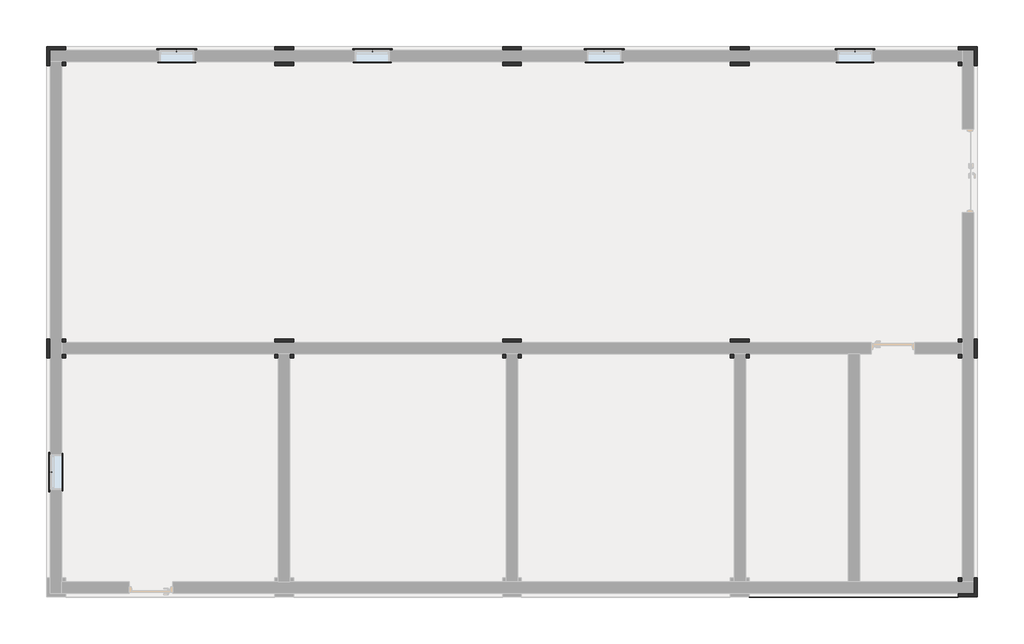
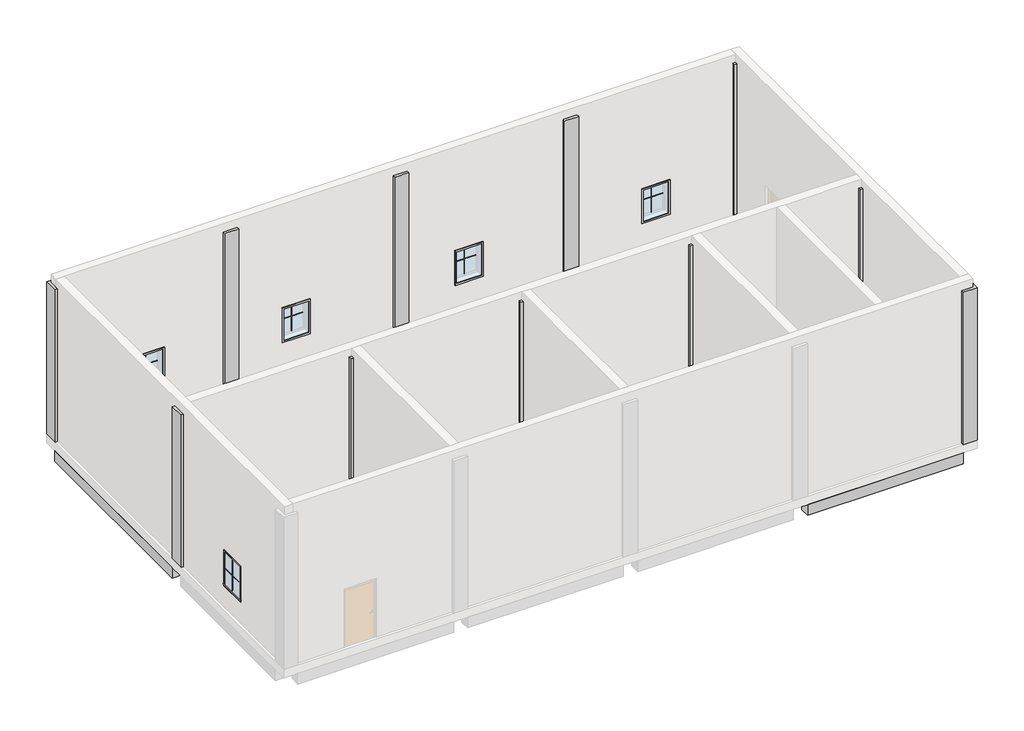
# One storey, part 2 of 2: 15 proxies, 11 columns, 8 beams.
"""IFC4 building model written with IfcOpenShell, lengths in millimetres."""

import ifcopenshell
import ifcopenshell.guid

model = None  # the IFC model being written
_history = None  # IfcOwnerHistory: only IFC2X3 demands one
_inside = {}  # id of a spatial element -> (the spatial element, [elements in it])
_under = {}  # id of a project, library or spatial element -> (it, [spatial elements below it])
_declared = {}  # id of a project -> (the project, [libraries it declares])
_typed = {}  # id of a type object -> (the type object, [elements of that type])
_made_of = {}  # id of a material, layer set ... -> (it, [elements and type objects made of it])


def new_model(schema):
    """Start an empty IFC model of exactly this schema.

    Asked for "IFC4X3", IfcOpenShell would pick the latest addendum, in which some entities
    have other attributes; the version numbers below select the first issue.
    IFC2X3 requires an IfcOwnerHistory on every rooted entity: one is made here for all.
    """
    global model, _history
    if schema == "IFC4X3":
        model = ifcopenshell.file(schema_version=(4, 3, 0, 0))
    else:
        model = ifcopenshell.file(schema=schema)
    _inside.clear()
    _under.clear()
    _declared.clear()
    _typed.clear()
    _made_of.clear()
    _history = None
    if model.schema == "IFC2X3":
        org = make("IfcOrganization", Name="unknown")
        user = make(
            "IfcPersonAndOrganization",
            ThePerson=make("IfcPerson", FamilyName="unknown"),
            TheOrganization=org,
        )
        app = make(
            "IfcApplication",
            ApplicationDeveloper=org,
            Version="unknown",
            ApplicationFullName="unknown",
            ApplicationIdentifier="unknown",
        )
        _history = make(
            "IfcOwnerHistory",
            OwningUser=user,
            OwningApplication=app,
            ChangeAction="ADDED",
            CreationDate=0,
        )
    return model


def make(cls, **values):
    """One entity of the class cls with the attributes given. An attribute that is None is left unset."""
    return model.create_entity(
        cls, **{name: value for name, value in values.items() if value is not None}
    )


def rooted(cls, **values):
    """An entity with a GlobalId (a new one), such as an element, a storey or a relation."""
    return make(cls, GlobalId=ifcopenshell.guid.new(), OwnerHistory=_history, **values)


def si_unit(unit_type, name, prefix=None):
    """IfcSIUnit, for example si_unit("LENGTHUNIT", "METRE", prefix="MILLI")."""
    return make("IfcSIUnit", UnitType=unit_type, Prefix=prefix, Name=name)


def assignment(units):
    """IfcUnitAssignment: the units of a project."""
    return None if units is None else make("IfcUnitAssignment", Units=units)


def point(xyz):
    """IfcCartesianPoint."""
    return None if xyz is None else make("IfcCartesianPoint", Coordinates=xyz)


def direction(xyz):
    """IfcDirection."""
    return None if xyz is None else make("IfcDirection", DirectionRatios=xyz)


def frame(location, z_axis=None, x_axis=None):
    """IfcAxis2Placement3D, a coordinate frame: its origin and axes. An axis left out is left unset."""
    return make(
        "IfcAxis2Placement3D",
        Location=point(location),
        Axis=direction(z_axis),
        RefDirection=direction(x_axis),
    )


def origin():
    """The frame at (0, 0, 0) with its axes left unset."""
    return frame((0.0, 0.0, 0.0))


def origin_with_axes():
    """The frame at (0, 0, 0) with the z axis (0, 0, 1) and the x axis (1, 0, 0) written out."""
    return frame((0.0, 0.0, 0.0), z_axis=(0.0, 0.0, 1.0), x_axis=(1.0, 0.0, 0.0))


def place(relative_to, where):
    """IfcLocalPlacement: puts the frame where relative to a parent placement (None: the world)."""
    return make(
        "IfcLocalPlacement", PlacementRelTo=relative_to, RelativePlacement=where
    )


def context(
    kind, dimensions, precision=None, world=None, true_north=None, identifier=None
):
    """IfcGeometricRepresentationContext, for example the 3D "Model" context."""
    return make(
        "IfcGeometricRepresentationContext",
        ContextIdentifier=identifier,
        ContextType=kind,
        CoordinateSpaceDimension=dimensions,
        Precision=precision,
        WorldCoordinateSystem=world,
        TrueNorth=true_north,
    )


def project(units=None, contexts=None):
    """IfcProject with its units and contexts."""
    return rooted(
        "IfcProject",
        Name="project",
        RepresentationContexts=contexts,
        UnitsInContext=assignment(units),
    )


def spatial(cls, under=None, at=None, **own):
    """A site, building, storey or space (cls), placed at a placement, below another one or the project."""
    s = rooted(cls, ObjectPlacement=at, **own)
    if under is not None:
        _under.setdefault(under.id(), (under, []))[1].append(s)
    return s


def polyline(points):
    """IfcPolyline through the points."""
    return make("IfcPolyline", Points=[point(p) for p in points])


def outline(outer, holes=None, kind="AREA"):
    """IfcArbitraryClosedProfileDef: a profile drawn as a closed curve; with holes, ...WithVoids."""
    if holes is None:
        return make("IfcArbitraryClosedProfileDef", ProfileType=kind, OuterCurve=outer)
    return make(
        "IfcArbitraryProfileDefWithVoids",
        ProfileType=kind,
        OuterCurve=outer,
        InnerCurves=holes,
    )


def extrude(swept, where, along, depth):
    """IfcExtrudedAreaSolid: the profile swept, set in the frame where, extruded along a direction by depth."""
    return make(
        "IfcExtrudedAreaSolid",
        SweptArea=swept,
        Position=where,
        ExtrudedDirection=direction(along),
        Depth=depth,
    )


def faces_of(points, faces, orient=None, outer=None):
    """IfcFace entities. A face is a list of loops; a loop is a list of indices into points, from 0.

    orient and outer hold one flag for each loop. By default every Orientation is true, the
    first loop of a face is its IfcFaceOuterBound and the others are IfcFaceBound.
    """
    made = []
    for i, loops in enumerate(faces):
        bounds = []
        for j, loop in enumerate(loops):
            is_outer = j == 0 if outer is None else outer[i][j]
            bounds.append(
                make(
                    "IfcFaceOuterBound" if is_outer else "IfcFaceBound",
                    Bound=make("IfcPolyLoop", Polygon=[points[k] for k in loop]),
                    Orientation=True if orient is None else orient[i][j],
                )
            )
        made.append(make("IfcFace", Bounds=bounds))
    return made


def faceted_brep(points, faces, orient=None, outer=None, voids=None):
    """IfcFacetedBrep: a solid bounded by flat faces; with voids (closed shells), ...WithVoids."""
    shared = [point(p) for p in points]
    hull = make("IfcClosedShell", CfsFaces=faces_of(shared, faces, orient, outer))
    if voids is None:
        return make("IfcFacetedBrep", Outer=hull)
    return make(
        "IfcFacetedBrepWithVoids",
        Outer=hull,
        Voids=[
            make(cls, CfsFaces=faces_of(shared, fs, o, b)) for cls, fs, o, b in voids
        ],
    )


def shape(context_of_items, identifier, shape_type, items):
    """IfcShapeRepresentation: the items that make up one representation, for example the "Body"."""
    return make(
        "IfcShapeRepresentation",
        ContextOfItems=context_of_items,
        RepresentationIdentifier=identifier,
        RepresentationType=shape_type,
        Items=items,
    )


def source(mapping_origin, context_of_items, identifier, shape_type, items):
    """IfcRepresentationMap: a shape defined once, which mapped items show again and again."""
    return make(
        "IfcRepresentationMap",
        MappingOrigin=mapping_origin,
        MappedRepresentation=shape(context_of_items, identifier, shape_type, items),
    )


def transform(
    local_origin,
    x_axis=None,
    y_axis=None,
    z_axis=None,
    scale=None,
    scale2=None,
    scale3=None,
    uniform=True,
):
    """IfcCartesianTransformationOperator3D, or its non-uniform kind. x_axis, y_axis, z_axis: its Axis1, 2, 3."""
    if uniform:
        return make(
            "IfcCartesianTransformationOperator3D",
            Axis1=direction(x_axis),
            Axis2=direction(y_axis),
            LocalOrigin=point(local_origin),
            Scale=scale,
            Axis3=direction(z_axis),
        )
    return make(
        "IfcCartesianTransformationOperator3DnonUniform",
        Axis1=direction(x_axis),
        Axis2=direction(y_axis),
        LocalOrigin=point(local_origin),
        Scale=scale,
        Axis3=direction(z_axis),
        Scale2=scale2,
        Scale3=scale3,
    )


def mapped(mapping_source, mapping_target):
    """IfcMappedItem: shows the shape of a source again, moved by a transform."""
    return make(
        "IfcMappedItem", MappingSource=mapping_source, MappingTarget=mapping_target
    )


def made_of(thing, what):
    """Note that an element or type object is made of a material, layer set ...; save() writes the relation."""
    if what is not None:
        _made_of.setdefault(what.id(), (what, []))[1].append(thing)
    return thing


def element(
    cls,
    number,
    at=None,
    inside=None,
    cuts=None,
    type_object=None,
    material=None,
    context=None,
    identifier="Body",
    shape_type=None,
    held_by="IfcProductDefinitionShape",
    body=None,
    shapes=None,
    **own,
):
    """One element of the class cls, such as IfcWall. Its Tag is "e" and its number.

    at: its placement. inside: the storey or other place that contains it. cuts: it is an
    opening in that element (IfcRelVoidsElement). A single representation is given by context,
    identifier, shape_type and body (its items); several are given by shapes. held_by: the class
    of the entity that holds the representations. save() writes the other relations.
    """
    e = rooted(cls, Tag="e%d" % number, ObjectPlacement=at, **own)
    if body is not None:
        shapes = [shape(context, identifier, shape_type, body)]
    if shapes is not None:
        e.Representation = make(held_by, Representations=shapes)
    if inside is not None:
        _inside.setdefault(inside.id(), (inside, []))[1].append(e)
    if cuts is not None:
        rooted(
            "IfcRelVoidsElement", RelatingBuildingElement=cuts, RelatedOpeningElement=e
        )
    if type_object is not None:
        _typed.setdefault(type_object.id(), (type_object, []))[1].append(e)
    return made_of(e, material)


def aggregate(whole, parts):
    """IfcRelAggregates: a whole, such as a stair, and the parts it consists of."""
    return rooted("IfcRelAggregates", RelatingObject=whole, RelatedObjects=parts)


def save(model, path):
    """Write the relations noted so far, then the file.

    IfcRelAggregates (storeys below a building ...), IfcRelContainedInSpatialStructure (elements
    in a storey), IfcRelDefinesByType, IfcRelAssociatesMaterial and IfcRelDeclares: one each for
    every whole, place, type object, material and project.
    """
    for whole, parts in _under.values():
        aggregate(whole, parts)
    for where, things in _inside.values():
        rooted(
            "IfcRelContainedInSpatialStructure",
            RelatedElements=things,
            RelatingStructure=where,
        )
    for kind, things in _typed.values():
        rooted("IfcRelDefinesByType", RelatedObjects=things, RelatingType=kind)
    for what, things in _made_of.values():
        rooted("IfcRelAssociatesMaterial", RelatedObjects=things, RelatingMaterial=what)
    for by, libraries in _declared.values():
        rooted("IfcRelDeclares", RelatingContext=by, RelatedDefinitions=libraries)
    model.write(path)


def m_muntin_pattern_2x2_m_muntin_pattern_2x2_ad852c99(model_context):
    return source(origin(), model_context, "Body", "SweptSolid", [
        extrude(outline(polyline([(568.25, -6.35), (568.25, -411.9), (555.55, -411.9), (555.55, -6.35), (0.0, -6.35), (0.0, 6.35), (555.55, 6.35), (555.55, 411.9), (568.25, 411.9), (568.25, 6.35), (1123.8, 6.35), (1123.8, -6.35), (568.25, -6.35)])), frame((0.0, -22.225, 0.0), z_axis=(0.0, 1.0, 0.0), x_axis=(0.0, 0.0, 1.0)), (0.0, 0.0, 1.0), 12.7),
        extrude(outline(polyline([(568.25, -6.35), (568.25, -411.9), (555.55, -411.9), (555.55, -6.35), (0.0, -6.35), (0.0, 6.35), (555.55, 6.35), (555.55, 411.9), (568.25, 411.9), (568.25, 6.35), (1123.8, 6.35), (1123.8, -6.35), (568.25, -6.35)])), frame((0.0, 9.525, 0.0), z_axis=(0.0, 1.0, 0.0), x_axis=(0.0, 0.0, 1.0)), (0.0, 0.0, 1.0), 12.7),
    ])


def m_trim_window_exterior_flat_with_sill_71544b40(model_context):
    return source(origin(), model_context, "Body", "SweptSolid", [
        extrude(outline(polyline([(510.0, -1220.4323709), (510.0, -1280.4323709), (-510.0, -1280.4323709), (-510.0, -1220.4323709), (510.0, -1220.4323709)])), origin_with_axes(), (0.0, 0.0, 1.0), 19.05),
        extrude(outline(polyline([(-1230.0, 38.1), (-1202.4580645, 38.1), (-1200.0, 19.05), (-1200.0, 0.0), (-1220.4323709, 0.0), (-1220.4323709, 19.05), (-1230.0, 19.05), (-1230.0, 38.1)])), frame((-522.7, 0.0, 0.0), z_axis=(1.0, 0.0, 0.0), x_axis=(0.0, 1.0, 0.0)), (0.0, 0.0, 1.0), 1045.4),
        extrude(outline(polyline([(-510.0, 60.0), (510.0, 60.0), (510.0, -1200.0), (450.0, -1200.0), (450.0, 0.0), (-450.0, 0.0), (-450.0, -1200.0), (-510.0, -1200.0), (-510.0, 60.0)])), origin_with_axes(), (0.0, 0.0, 1.0), 19.05),
    ])


def m_trim_window_interior_flat_picture_frame_24fe8ef8(model_context):
    return source(origin(), model_context, "Body", "SweptSolid", [
        extrude(outline(polyline([(497.3, 47.3), (497.3, -1247.3), (-497.3, -1247.3), (-497.3, 47.3), (497.3, 47.3)]), holes=[polyline([(437.3, -12.7), (-437.3, -12.7), (-437.3, -1187.3), (437.3, -1187.3), (437.3, -12.7)])]), origin_with_axes(), (0.0, 0.0, 1.0), 30.0),
    ])


model = new_model("IFC4")

# Units and contexts
model_context = context("Model", 3, world=origin())
ifc_project = project(units=[si_unit("LENGTHUNIT", "METRE", prefix="MILLI")], contexts=[model_context])

# Site, building, storey
site = spatial("IfcSite", under=ifc_project)
building = spatial("IfcBuilding", under=site)
storey = spatial("IfcBuildingStorey", under=building, Name="1st FL GL+200", Elevation=0.0)

# Beams
placement = place(None, origin())
element("IfcBeam", 1, ObjectType="RC Beam_Rectangular : 350 x 700mm", at=placement, inside=storey, context=model_context, shape_type="SweptSolid", body=[
    extrude(outline(polyline([(5204.2726763, 1485.9763125), (5554.2726763, 1485.9763125), (5554.2726763, -4314.0236875), (5204.2726763, -4314.0236875), (5204.2726763, 1485.9763125)])), frame((0.0, 0.0, -700.0), z_axis=(0.0, 0.0, 1.0), x_axis=(1.0, 0.0, 0.0)), (0.0, 0.0, 1.0), 400.0),
])
element("IfcBeam", 2, ObjectType="RC Beam_Rectangular : 350 x 700mm", at=placement, inside=storey, context=model_context, shape_type="SweptSolid", body=[
    extrude(outline(polyline([(5554.2726763, 1998.6763125), (5204.2726763, 1998.6763125), (5204.2726763, 9185.9763125), (5554.2726763, 9185.9763125), (5554.2726763, 1998.6763125)])), frame((0.0, 0.0, -700.0), z_axis=(0.0, 0.0, 1.0), x_axis=(1.0, 0.0, 0.0)), (0.0, 0.0, 1.0), 400.0),
])
element("IfcBeam", 3, ObjectType="RC Beam_Rectangular : 350 x 700mm", at=placement, inside=storey, context=model_context, shape_type="SweptSolid", body=[
    extrude(outline(polyline([(-18595.7273237, 1998.6763125), (-18945.7273237, 1998.6763125), (-18945.7273237, 9185.9763125), (-18595.7273237, 9185.9763125), (-18595.7273237, 1998.6763125)])), frame((0.0, 0.0, -700.0), z_axis=(0.0, 0.0, 1.0), x_axis=(1.0, 0.0, 0.0)), (0.0, 0.0, 1.0), 400.0),
])
element("IfcBeam", 4, ObjectType="RC Beam_Rectangular : 350 x 700mm", at=placement, inside=storey, context=model_context, shape_type="SweptSolid", body=[
    extrude(outline(polyline([(-12945.7273237, 9685.9763125), (-12945.7273237, 9335.9763125), (-18445.7273237, 9335.9763125), (-18445.7273237, 9685.9763125), (-12945.7273237, 9685.9763125)])), frame((0.0, 0.0, -700.0), z_axis=(0.0, 0.0, 1.0), x_axis=(1.0, 0.0, 0.0)), (0.0, 0.0, 1.0), 400.0),
])
element("IfcBeam", 5, ObjectType="RC Beam_Rectangular : 350 x 700mm", at=placement, inside=storey, context=model_context, shape_type="SweptSolid", body=[
    extrude(outline(polyline([(-12433.0273237, 9335.9763125), (-12433.0273237, 9685.9763125), (-6945.7273237, 9685.9763125), (-6945.7273237, 9335.9763125), (-12433.0273237, 9335.9763125)])), frame((0.0, 0.0, -700.0), z_axis=(0.0, 0.0, 1.0), x_axis=(1.0, 0.0, 0.0)), (0.0, 0.0, 1.0), 400.0),
])
element("IfcBeam", 6, ObjectType="RC Beam_Rectangular : 350 x 700mm", at=placement, inside=storey, context=model_context, shape_type="SweptSolid", body=[
    extrude(outline(polyline([(-6433.0273237, 9335.9763125), (-6433.0273237, 9685.9763125), (-945.7273237, 9685.9763125), (-945.7273237, 9335.9763125), (-6433.0273237, 9335.9763125)])), frame((0.0, 0.0, -700.0), z_axis=(0.0, 0.0, 1.0), x_axis=(1.0, 0.0, 0.0)), (0.0, 0.0, 1.0), 400.0),
])
element("IfcBeam", 7, ObjectType="RC Beam_Rectangular : 350 x 700mm", at=placement, inside=storey, context=model_context, shape_type="SweptSolid", body=[
    extrude(outline(polyline([(-433.0273237, 9335.9763125), (-433.0273237, 9685.9763125), (5054.2726763, 9685.9763125), (5054.2726763, 9335.9763125), (-433.0273237, 9335.9763125)])), frame((0.0, 0.0, -700.0), z_axis=(0.0, 0.0, 1.0), x_axis=(1.0, 0.0, 0.0)), (0.0, 0.0, 1.0), 400.0),
])
element("IfcBeam", 8, ObjectType="RC Beam_Rectangular : 350 x 700mm", at=placement, inside=storey, context=model_context, shape_type="SweptSolid", body=[
    extrude(outline(polyline([(5054.2726763, -4464.0236875), (5054.2726763, -4814.0236875), (-445.7273237, -4814.0236875), (-445.7273237, -4464.0236875), (5054.2726763, -4464.0236875)])), frame((0.0, 0.0, -700.0), z_axis=(0.0, 0.0, 1.0), x_axis=(1.0, 0.0, 0.0)), (0.0, 0.0, 1.0), 400.0),
])

# Proxies
m_muntin_pattern_2x2_m_muntin_pattern_2x2_shape = m_muntin_pattern_2x2_m_muntin_pattern_2x2_ad852c99(model_context)
element("IfcBuildingElementProxy", 9, Name="M_Muntin Pattern_2x2 : M_Muntin Pattern_2x2", ObjectType="M_Muntin Pattern_2x2 : M_Muntin Pattern_2x2", at=placement, inside=storey, context=model_context, shape_type="MappedRepresentation", body=[
    mapped(m_muntin_pattern_2x2_m_muntin_pattern_2x2_shape, transform((2329.2726763, 9576.4513125, 938.1), x_axis=(-1.0, 0.0, 0.0), y_axis=(0.0, -1.0, 0.0), z_axis=(0.0, 0.0, 1.0))),
])
element("IfcBuildingElementProxy", 10, Name="M_Muntin Pattern_2x2 : M_Muntin Pattern_2x2", ObjectType="M_Muntin Pattern_2x2 : M_Muntin Pattern_2x2", at=placement, inside=storey, context=model_context, shape_type="MappedRepresentation", body=[
    mapped(m_muntin_pattern_2x2_m_muntin_pattern_2x2_shape, transform((-4270.7273237, 9576.4513125, 938.1), x_axis=(-1.0, 0.0, 0.0), y_axis=(0.0, -1.0, 0.0), z_axis=(0.0, 0.0, 1.0))),
])
element("IfcBuildingElementProxy", 11, Name="M_Muntin Pattern_2x2 : M_Muntin Pattern_2x2", ObjectType="M_Muntin Pattern_2x2 : M_Muntin Pattern_2x2", at=placement, inside=storey, context=model_context, shape_type="MappedRepresentation", body=[
    mapped(m_muntin_pattern_2x2_m_muntin_pattern_2x2_shape, transform((-10370.7273237, 9576.4513125, 938.1), x_axis=(-1.0, 0.0, 0.0), y_axis=(0.0, -1.0, 0.0), z_axis=(0.0, 0.0, 1.0))),
])
element("IfcBuildingElementProxy", 12, Name="M_Muntin Pattern_2x2 : M_Muntin Pattern_2x2", ObjectType="M_Muntin Pattern_2x2 : M_Muntin Pattern_2x2", at=placement, inside=storey, context=model_context, shape_type="MappedRepresentation", body=[
    mapped(m_muntin_pattern_2x2_m_muntin_pattern_2x2_shape, transform((-15520.7273237, 9576.4513125, 938.1), x_axis=(-1.0, 0.0, 0.0), y_axis=(0.0, -1.0, 0.0), z_axis=(0.0, 0.0, 1.0))),
])
element("IfcBuildingElementProxy", 13, Name="M_Muntin Pattern_2x2 : M_Muntin Pattern_2x2", ObjectType="M_Muntin Pattern_2x2 : M_Muntin Pattern_2x2", at=placement, inside=storey, context=model_context, shape_type="MappedRepresentation", body=[
    mapped(m_muntin_pattern_2x2_m_muntin_pattern_2x2_shape, transform((-18836.2023237, -1526.5236875, 938.1), x_axis=(0.0, -1.0, 0.0), y_axis=(1.0, 0.0, 0.0), z_axis=(0.0, 0.0, 1.0))),
])
m_trim_window_exterior_flat_with_sill_shape = m_trim_window_exterior_flat_with_sill_71544b40(model_context)
element("IfcBuildingElementProxy", 14, Name="M_Trim-Window-Exterior-Flat : with Sill", ObjectType="M_Trim-Window-Exterior-Flat : with Sill", at=placement, inside=storey, context=model_context, shape_type="MappedRepresentation", body=[
    mapped(m_trim_window_exterior_flat_with_sill_shape, transform((2329.2726763, 9585.9763125, 2100.0), x_axis=(-1.0, 0.0, 0.0), y_axis=(0.0, 0.0, 1.0), z_axis=(0.0, 1.0, 0.0))),
])
element("IfcBuildingElementProxy", 15, Name="M_Trim-Window-Exterior-Flat : with Sill", ObjectType="M_Trim-Window-Exterior-Flat : with Sill", at=placement, inside=storey, context=model_context, shape_type="MappedRepresentation", body=[
    mapped(m_trim_window_exterior_flat_with_sill_shape, transform((-4270.7273237, 9585.9763125, 2100.0), x_axis=(-1.0, 0.0, 0.0), y_axis=(0.0, 0.0, 1.0), z_axis=(0.0, 1.0, 0.0))),
])
element("IfcBuildingElementProxy", 16, Name="M_Trim-Window-Exterior-Flat : with Sill", ObjectType="M_Trim-Window-Exterior-Flat : with Sill", at=placement, inside=storey, context=model_context, shape_type="MappedRepresentation", body=[
    mapped(m_trim_window_exterior_flat_with_sill_shape, transform((-10370.7273237, 9585.9763125, 2100.0), x_axis=(-1.0, 0.0, 0.0), y_axis=(0.0, 0.0, 1.0), z_axis=(0.0, 1.0, 0.0))),
])
element("IfcBuildingElementProxy", 17, Name="M_Trim-Window-Exterior-Flat : with Sill", ObjectType="M_Trim-Window-Exterior-Flat : with Sill", at=placement, inside=storey, context=model_context, shape_type="MappedRepresentation", body=[
    mapped(m_trim_window_exterior_flat_with_sill_shape, transform((-15520.7273237, 9585.9763125, 2100.0), x_axis=(-1.0, 0.0, 0.0), y_axis=(0.0, 0.0, 1.0), z_axis=(0.0, 1.0, 0.0))),
])
element("IfcBuildingElementProxy", 18, Name="M_Trim-Window-Exterior-Flat : with Sill", ObjectType="M_Trim-Window-Exterior-Flat : with Sill", at=placement, inside=storey, context=model_context, shape_type="MappedRepresentation", body=[
    mapped(m_trim_window_exterior_flat_with_sill_shape, transform((-18845.7273237, -1526.5236875, 2100.0), x_axis=(0.0, -1.0, 0.0), y_axis=(0.0, 0.0, 1.0), z_axis=(-1.0, 0.0, 0.0))),
])
m_trim_window_interior_flat_picture_frame_shape = m_trim_window_interior_flat_picture_frame_24fe8ef8(model_context)
element("IfcBuildingElementProxy", 19, Name="M_Trim-Window-Interior-Flat : Picture Frame", ObjectType="M_Trim-Window-Interior-Flat : Picture Frame", at=placement, inside=storey, context=model_context, shape_type="MappedRepresentation", body=[
    mapped(m_trim_window_interior_flat_picture_frame_shape, transform((2329.2726763, 9285.9763125, 2100.0), x_axis=(1.0, 0.0, 0.0), y_axis=(0.0, 0.0, 1.0), z_axis=(0.0, -1.0, 0.0))),
])
element("IfcBuildingElementProxy", 20, Name="M_Trim-Window-Interior-Flat : Picture Frame", ObjectType="M_Trim-Window-Interior-Flat : Picture Frame", at=placement, inside=storey, context=model_context, shape_type="MappedRepresentation", body=[
    mapped(m_trim_window_interior_flat_picture_frame_shape, transform((-4270.7273237, 9285.9763125, 2100.0), x_axis=(1.0, 0.0, 0.0), y_axis=(0.0, 0.0, 1.0), z_axis=(0.0, -1.0, 0.0))),
])
element("IfcBuildingElementProxy", 21, Name="M_Trim-Window-Interior-Flat : Picture Frame", ObjectType="M_Trim-Window-Interior-Flat : Picture Frame", at=placement, inside=storey, context=model_context, shape_type="MappedRepresentation", body=[
    mapped(m_trim_window_interior_flat_picture_frame_shape, transform((-10370.7273237, 9285.9763125, 2100.0), x_axis=(1.0, 0.0, 0.0), y_axis=(0.0, 0.0, 1.0), z_axis=(0.0, -1.0, 0.0))),
])
element("IfcBuildingElementProxy", 22, Name="M_Trim-Window-Interior-Flat : Picture Frame", ObjectType="M_Trim-Window-Interior-Flat : Picture Frame", at=placement, inside=storey, context=model_context, shape_type="MappedRepresentation", body=[
    mapped(m_trim_window_interior_flat_picture_frame_shape, transform((-15520.7273237, 9285.9763125, 2100.0), x_axis=(1.0, 0.0, 0.0), y_axis=(0.0, 0.0, 1.0), z_axis=(0.0, -1.0, 0.0))),
])
element("IfcBuildingElementProxy", 23, Name="M_Trim-Window-Interior-Flat : Picture Frame", ObjectType="M_Trim-Window-Interior-Flat : Picture Frame", at=placement, inside=storey, context=model_context, shape_type="MappedRepresentation", body=[
    mapped(m_trim_window_interior_flat_picture_frame_shape, transform((-18545.7273237, -1526.5236875, 2100.0), x_axis=(0.0, 1.0, 0.0), y_axis=(0.0, 0.0, 1.0), z_axis=(1.0, 0.0, 0.0))),
])

# Columns
element("IfcColumn", 24, ObjectType="RC_Column_Rectangular : 500 x 500mm", at=placement, inside=storey, context=model_context, shape_type="Brep", body=[
    faceted_brep([(-18945.7273237, 9185.9763125, 0.0), (-18945.7273237, 9685.9763125, 0.0), (-18445.7273237, 9685.9763125, 0.0), (-18445.7273237, 9585.9763125, 0.0), (-18845.7273237, 9585.9763125, 0.0), (-18845.7273237, 9285.9763125, 0.0), (-18845.7273237, 9185.9763125, 0.0), (-18945.7273237, 9685.9763125, 5700.0), (-18445.7273237, 9685.9763125, 5700.0), (-18445.7273237, 9685.9763125, 5300.0), (-18945.7273237, 9185.9763125, 5300.0), (-18945.7273237, 9185.9763125, 5700.0), (-18845.7273237, 9185.9763125, 5300.0), (-18845.7273237, 9185.9763125, 5700.0), (-18445.7273237, 9585.9763125, 5700.0), (-18445.7273237, 9585.9763125, 5300.0), (-18845.7273237, 9585.9763125, 5700.0)], [[[0, 1, 2, 3, 4, 5, 6]], [[2, 1, 7, 8, 9]], [[1, 0, 10, 11, 7]], [[11, 10, 0, 6, 12, 13]], [[2, 9, 8, 14, 15, 3]], [[16, 4, 3, 15, 14]], [[4, 16, 13, 12, 6, 5]], [[8, 7, 11, 13, 16, 14]]]),
    faceted_brep([(-18445.7273237, 9185.9763125, 5700.0), (-18445.7273237, 9285.9763125, 5700.0), (-18545.7273237, 9285.9763125, 5700.0), (-18545.7273237, 9185.9763125, 5700.0), (-18445.7273237, 9285.9763125, 0.0), (-18545.7273237, 9285.9763125, 0.0), (-18445.7273237, 9185.9763125, 0.0), (-18545.7273237, 9185.9763125, 0.0)], [[[0, 1, 2, 3]], [[1, 4, 5, 2]], [[0, 6, 4, 1]], [[5, 7, 3, 2]], [[4, 6, 7, 5]], [[6, 0, 3, 7]]]),
])
element("IfcColumn", 25, ObjectType="RC_Column_Rectangular : 500 x 500mm", at=placement, inside=storey, context=model_context, shape_type="Brep", body=[
    faceted_brep([(-18945.7273237, 1485.9763125, 0.0), (-18945.7273237, 1985.9763125, 0.0), (-18845.7273237, 1985.9763125, 0.0), (-18845.7273237, 1485.9763125, 0.0), (-18945.7273237, 1485.9763125, 5300.0), (-18945.7273237, 1485.9763125, 5700.0), (-18945.7273237, 1985.9763125, 5700.0), (-18945.7273237, 1985.9763125, 5300.0), (-18845.7273237, 1485.9763125, 5300.0), (-18845.7273237, 1485.9763125, 5700.0), (-18845.7273237, 1985.9763125, 5300.0), (-18845.7273237, 1985.9763125, 5700.0)], [[[0, 1, 2, 3]], [[1, 0, 4, 5, 6, 7]], [[5, 4, 0, 3, 8, 9]], [[3, 2, 10, 11, 9, 8]], [[1, 7, 6, 11, 10, 2]], [[6, 5, 9, 11]]]),
    faceted_brep([(-18445.7273237, 1985.9763125, 5700.0), (-18445.7273237, 1985.9763125, 0.0), (-18545.7273237, 1985.9763125, 0.0), (-18545.7273237, 1985.9763125, 5700.0), (-18445.7273237, 1910.9763125, 5700.0), (-18445.7273237, 1885.9763125, 5700.0), (-18445.7273237, 1885.9763125, 5300.0), (-18445.7273237, 1885.9763125, 0.0), (-18545.7273237, 1885.9763125, 0.0), (-18545.7273237, 1885.9763125, 5700.0)], [[[0, 1, 2, 3]], [[1, 0, 4, 5, 6, 7]], [[2, 1, 7, 8]], [[7, 6, 5, 9, 8]], [[0, 3, 9, 5, 4]], [[3, 2, 8, 9]]]),
    faceted_brep([(-18545.7273237, 1485.9763125, 5700.0), (-18445.7273237, 1485.9763125, 5700.0), (-18445.7273237, 1560.9763125, 5700.0), (-18445.7273237, 1585.9763125, 5700.0), (-18545.7273237, 1585.9763125, 5700.0), (-18545.7273237, 1485.9763125, 0.0), (-18545.7273237, 1585.9763125, 0.0), (-18445.7273237, 1485.9763125, 0.0), (-18445.7273237, 1585.9763125, 5300.0), (-18445.7273237, 1585.9763125, 0.0)], [[[0, 1, 2, 3, 4]], [[5, 0, 4, 6]], [[7, 1, 0, 5]], [[3, 8, 9, 6, 4]], [[1, 7, 9, 8, 3, 2]], [[7, 5, 6, 9]]]),
])
element("IfcColumn", 26, ObjectType="RC_Column_Rectangular : 500 x 500mm", at=placement, inside=storey, context=model_context, shape_type="Brep", body=[
    faceted_brep([(-12945.7273237, 9685.9763125, 0.0), (-12445.7273237, 9685.9763125, 0.0), (-12445.7273237, 9585.9763125, 0.0), (-12945.7273237, 9585.9763125, 0.0), (-12945.7273237, 9685.9763125, 5300.0), (-12945.7273237, 9685.9763125, 5700.0), (-12445.7273237, 9685.9763125, 5700.0), (-12945.7273237, 9585.9763125, 5300.0), (-12945.7273237, 9585.9763125, 5700.0), (-12445.7273237, 9585.9763125, 5700.0)], [[[0, 1, 2, 3]], [[1, 0, 4, 5, 6]], [[5, 4, 0, 3, 7, 8]], [[1, 6, 9, 2]], [[3, 2, 9, 8, 7]], [[6, 5, 8, 9]]]),
    faceted_brep([(-12945.7273237, 9185.9763125, 0.0), (-12445.7273237, 9185.9763125, 0.0), (-12445.7273237, 9185.9763125, 5700.0), (-12520.7273237, 9185.9763125, 5700.0), (-12870.7273237, 9185.9763125, 5700.0), (-12945.7273237, 9185.9763125, 5700.0), (-12445.7273237, 9285.9763125, 5700.0), (-12945.7273237, 9285.9763125, 5700.0), (-12445.7273237, 9285.9763125, 0.0), (-12945.7273237, 9285.9763125, 0.0)], [[[0, 1, 2, 3, 4, 5]], [[5, 4, 3, 2, 6, 7]], [[8, 9, 7, 6]], [[1, 0, 9, 8]], [[0, 5, 7, 9]], [[2, 1, 8, 6]]]),
])
element("IfcColumn", 27, ObjectType="RC_Column_Rectangular : 500 x 500mm", at=placement, inside=storey, context=model_context, shape_type="Brep", body=[
    faceted_brep([(-12945.7273237, 1985.9763125, 0.0), (-12445.7273237, 1985.9763125, 0.0), (-12445.7273237, 1885.9763125, 0.0), (-12945.7273237, 1885.9763125, 0.0), (-12945.7273237, 1985.9763125, 5700.0), (-12870.7273237, 1985.9763125, 5700.0), (-12520.7273237, 1985.9763125, 5700.0), (-12445.7273237, 1985.9763125, 5700.0), (-12945.7273237, 1885.9763125, 5300.0), (-12945.7273237, 1885.9763125, 5700.0), (-12945.7273237, 1910.9763125, 5700.0), (-12445.7273237, 1910.9763125, 5700.0), (-12445.7273237, 1885.9763125, 5700.0), (-12445.7273237, 1885.9763125, 5300.0)], [[[0, 1, 2, 3]], [[1, 0, 4, 5, 6, 7]], [[4, 0, 3, 8, 9, 10]], [[1, 7, 11, 12, 13, 2]], [[3, 2, 13, 12, 9, 8]], [[7, 6, 5, 4, 10, 9, 12, 11]]]),
    faceted_brep([(-12945.7273237, 1485.9763125, 5700.0), (-12945.7273237, 1485.9763125, 0.0), (-12845.7273237, 1485.9763125, 0.0), (-12845.7273237, 1485.9763125, 5300.0), (-12845.7273237, 1485.9763125, 5700.0), (-12870.7273237, 1485.9763125, 5700.0), (-12945.7273237, 1585.9763125, 0.0), (-12945.7273237, 1585.9763125, 5300.0), (-12945.7273237, 1585.9763125, 5700.0), (-12845.7273237, 1585.9763125, 5700.0), (-12845.7273237, 1585.9763125, 0.0), (-12945.7273237, 1560.9763125, 5700.0)], [[[0, 1, 2, 3, 4, 5]], [[6, 7, 8, 9, 10]], [[1, 6, 10, 2]], [[1, 0, 11, 8, 7, 6]], [[4, 3, 2, 10, 9]], [[8, 11, 0, 5, 4, 9]]]),
    faceted_brep([(-12445.7273237, 1485.9763125, 5700.0), (-12445.7273237, 1560.9763125, 5700.0), (-12445.7273237, 1585.9763125, 5700.0), (-12545.7273237, 1585.9763125, 5700.0), (-12545.7273237, 1485.9763125, 5700.0), (-12520.7273237, 1485.9763125, 5700.0), (-12445.7273237, 1485.9763125, 0.0), (-12445.7273237, 1585.9763125, 0.0), (-12445.7273237, 1585.9763125, 5300.0), (-12545.7273237, 1485.9763125, 0.0), (-12545.7273237, 1485.9763125, 5300.0), (-12545.7273237, 1585.9763125, 0.0)], [[[0, 1, 2, 3, 4, 5]], [[0, 6, 7, 8, 2, 1]], [[9, 10, 4, 3, 11]], [[6, 0, 5, 4, 10, 9]], [[2, 8, 7, 11, 3]], [[7, 6, 9, 11]]]),
])
element("IfcColumn", 28, ObjectType="RC_Column_Rectangular : 500 x 500mm", at=placement, inside=storey, context=model_context, shape_type="Brep", body=[
    faceted_brep([(-6945.7273237, 9685.9763125, 0.0), (-6445.7273237, 9685.9763125, 0.0), (-6445.7273237, 9585.9763125, 0.0), (-6945.7273237, 9585.9763125, 0.0), (-6945.7273237, 9685.9763125, 5300.0), (-6945.7273237, 9685.9763125, 5700.0), (-6445.7273237, 9685.9763125, 5700.0), (-6945.7273237, 9585.9763125, 5300.0), (-6945.7273237, 9585.9763125, 5700.0), (-6445.7273237, 9585.9763125, 5700.0)], [[[0, 1, 2, 3]], [[1, 0, 4, 5, 6]], [[5, 4, 0, 3, 7, 8]], [[1, 6, 9, 2]], [[3, 2, 9, 8, 7]], [[6, 5, 8, 9]]]),
    faceted_brep([(-6945.7273237, 9185.9763125, 0.0), (-6445.7273237, 9185.9763125, 0.0), (-6445.7273237, 9185.9763125, 5700.0), (-6520.7273237, 9185.9763125, 5700.0), (-6870.7273237, 9185.9763125, 5700.0), (-6945.7273237, 9185.9763125, 5700.0), (-6445.7273237, 9285.9763125, 5700.0), (-6945.7273237, 9285.9763125, 5700.0), (-6445.7273237, 9285.9763125, 0.0), (-6945.7273237, 9285.9763125, 0.0)], [[[0, 1, 2, 3, 4, 5]], [[5, 4, 3, 2, 6, 7]], [[8, 9, 7, 6]], [[1, 0, 9, 8]], [[0, 5, 7, 9]], [[2, 1, 8, 6]]]),
])
element("IfcColumn", 29, ObjectType="RC_Column_Rectangular : 500 x 500mm", at=placement, inside=storey, context=model_context, shape_type="Brep", body=[
    faceted_brep([(-6945.7273237, 1985.9763125, 0.0), (-6445.7273237, 1985.9763125, 0.0), (-6445.7273237, 1885.9763125, 0.0), (-6945.7273237, 1885.9763125, 0.0), (-6945.7273237, 1985.9763125, 5700.0), (-6870.7273237, 1985.9763125, 5700.0), (-6520.7273237, 1985.9763125, 5700.0), (-6445.7273237, 1985.9763125, 5700.0), (-6945.7273237, 1885.9763125, 5300.0), (-6945.7273237, 1885.9763125, 5700.0), (-6945.7273237, 1910.9763125, 5700.0), (-6445.7273237, 1910.9763125, 5700.0), (-6445.7273237, 1885.9763125, 5700.0), (-6445.7273237, 1885.9763125, 5300.0)], [[[0, 1, 2, 3]], [[1, 0, 4, 5, 6, 7]], [[4, 0, 3, 8, 9, 10]], [[1, 7, 11, 12, 13, 2]], [[3, 2, 13, 12, 9, 8]], [[7, 6, 5, 4, 10, 9, 12, 11]]]),
    faceted_brep([(-6945.7273237, 1485.9763125, 5700.0), (-6945.7273237, 1485.9763125, 0.0), (-6845.7273237, 1485.9763125, 0.0), (-6845.7273237, 1485.9763125, 5300.0), (-6845.7273237, 1485.9763125, 5700.0), (-6870.7273237, 1485.9763125, 5700.0), (-6945.7273237, 1585.9763125, 0.0), (-6945.7273237, 1585.9763125, 5300.0), (-6945.7273237, 1585.9763125, 5700.0), (-6845.7273237, 1585.9763125, 5700.0), (-6845.7273237, 1585.9763125, 0.0), (-6945.7273237, 1560.9763125, 5700.0)], [[[0, 1, 2, 3, 4, 5]], [[6, 7, 8, 9, 10]], [[1, 6, 10, 2]], [[1, 0, 11, 8, 7, 6]], [[4, 3, 2, 10, 9]], [[8, 11, 0, 5, 4, 9]]]),
    faceted_brep([(-6445.7273237, 1485.9763125, 5700.0), (-6445.7273237, 1560.9763125, 5700.0), (-6445.7273237, 1585.9763125, 5700.0), (-6545.7273237, 1585.9763125, 5700.0), (-6545.7273237, 1485.9763125, 5700.0), (-6520.7273237, 1485.9763125, 5700.0), (-6445.7273237, 1485.9763125, 0.0), (-6445.7273237, 1585.9763125, 0.0), (-6445.7273237, 1585.9763125, 5300.0), (-6545.7273237, 1485.9763125, 0.0), (-6545.7273237, 1485.9763125, 5300.0), (-6545.7273237, 1585.9763125, 0.0)], [[[0, 1, 2, 3, 4, 5]], [[0, 6, 7, 8, 2, 1]], [[9, 10, 4, 3, 11]], [[6, 0, 5, 4, 10, 9]], [[2, 8, 7, 11, 3]], [[7, 6, 9, 11]]]),
])
element("IfcColumn", 30, ObjectType="RC_Column_Rectangular : 500 x 500mm", at=placement, inside=storey, context=model_context, shape_type="Brep", body=[
    faceted_brep([(-945.7273237, 9685.9763125, 0.0), (-445.7273237, 9685.9763125, 0.0), (-445.7273237, 9585.9763125, 0.0), (-945.7273237, 9585.9763125, 0.0), (-945.7273237, 9685.9763125, 5300.0), (-945.7273237, 9685.9763125, 5700.0), (-445.7273237, 9685.9763125, 5700.0), (-945.7273237, 9585.9763125, 5300.0), (-945.7273237, 9585.9763125, 5700.0), (-445.7273237, 9585.9763125, 5700.0)], [[[0, 1, 2, 3]], [[1, 0, 4, 5, 6]], [[5, 4, 0, 3, 7, 8]], [[1, 6, 9, 2]], [[3, 2, 9, 8, 7]], [[6, 5, 8, 9]]]),
    faceted_brep([(-945.7273237, 9185.9763125, 0.0), (-445.7273237, 9185.9763125, 0.0), (-445.7273237, 9185.9763125, 5700.0), (-520.7273237, 9185.9763125, 5700.0), (-870.7273237, 9185.9763125, 5700.0), (-945.7273237, 9185.9763125, 5700.0), (-445.7273237, 9285.9763125, 5700.0), (-945.7273237, 9285.9763125, 5700.0), (-445.7273237, 9285.9763125, 0.0), (-945.7273237, 9285.9763125, 0.0)], [[[0, 1, 2, 3, 4, 5]], [[5, 4, 3, 2, 6, 7]], [[8, 9, 7, 6]], [[1, 0, 9, 8]], [[0, 5, 7, 9]], [[2, 1, 8, 6]]]),
])
element("IfcColumn", 31, ObjectType="RC_Column_Rectangular : 500 x 500mm", at=placement, inside=storey, context=model_context, shape_type="Brep", body=[
    faceted_brep([(-945.7273237, 1985.9763125, 0.0), (-445.7273237, 1985.9763125, 0.0), (-445.7273237, 1885.9763125, 0.0), (-945.7273237, 1885.9763125, 0.0), (-945.7273237, 1985.9763125, 5700.0), (-870.7273237, 1985.9763125, 5700.0), (-520.7273237, 1985.9763125, 5700.0), (-445.7273237, 1985.9763125, 5700.0), (-945.7273237, 1885.9763125, 5300.0), (-945.7273237, 1885.9763125, 5700.0), (-945.7273237, 1910.9763125, 5700.0), (-445.7273237, 1910.9763125, 5700.0), (-445.7273237, 1885.9763125, 5700.0), (-445.7273237, 1885.9763125, 5300.0)], [[[0, 1, 2, 3]], [[1, 0, 4, 5, 6, 7]], [[4, 0, 3, 8, 9, 10]], [[1, 7, 11, 12, 13, 2]], [[3, 2, 13, 12, 9, 8]], [[7, 6, 5, 4, 10, 9, 12, 11]]]),
    faceted_brep([(-945.7273237, 1485.9763125, 5700.0), (-945.7273237, 1485.9763125, 0.0), (-845.7273237, 1485.9763125, 0.0), (-845.7273237, 1485.9763125, 5300.0), (-845.7273237, 1485.9763125, 5700.0), (-870.7273237, 1485.9763125, 5700.0), (-945.7273237, 1585.9763125, 0.0), (-945.7273237, 1585.9763125, 5300.0), (-945.7273237, 1585.9763125, 5700.0), (-845.7273237, 1585.9763125, 5700.0), (-845.7273237, 1585.9763125, 0.0), (-945.7273237, 1560.9763125, 5700.0)], [[[0, 1, 2, 3, 4, 5]], [[6, 7, 8, 9, 10]], [[1, 6, 10, 2]], [[1, 0, 11, 8, 7, 6]], [[4, 3, 2, 10, 9]], [[8, 11, 0, 5, 4, 9]]]),
    faceted_brep([(-445.7273237, 1485.9763125, 5700.0), (-445.7273237, 1560.9763125, 5700.0), (-445.7273237, 1585.9763125, 5700.0), (-545.7273237, 1585.9763125, 5700.0), (-545.7273237, 1485.9763125, 5700.0), (-520.7273237, 1485.9763125, 5700.0), (-445.7273237, 1485.9763125, 0.0), (-445.7273237, 1585.9763125, 0.0), (-445.7273237, 1585.9763125, 5300.0), (-545.7273237, 1485.9763125, 0.0), (-545.7273237, 1485.9763125, 5300.0), (-545.7273237, 1585.9763125, 0.0)], [[[0, 1, 2, 3, 4, 5]], [[0, 6, 7, 8, 2, 1]], [[9, 10, 4, 3, 11]], [[6, 0, 5, 4, 10, 9]], [[2, 8, 7, 11, 3]], [[7, 6, 9, 11]]]),
])
element("IfcColumn", 32, ObjectType="RC_Column_Rectangular : 500 x 500mm", at=placement, inside=storey, context=model_context, shape_type="Brep", body=[
    faceted_brep([(5054.2726763, 9185.9763125, 0.0), (5054.2726763, 9285.9763125, 0.0), (5154.2726763, 9285.9763125, 0.0), (5154.2726763, 9185.9763125, 0.0), (5054.2726763, 9185.9763125, 5700.0), (5154.2726763, 9185.9763125, 5700.0), (5054.2726763, 9285.9763125, 5700.0), (5154.2726763, 9285.9763125, 5700.0)], [[[0, 1, 2, 3]], [[4, 0, 3, 5]], [[6, 4, 5, 7]], [[2, 1, 6, 7]], [[0, 4, 6, 1]], [[3, 2, 7, 5]]]),
    faceted_brep([(5554.2726763, 9685.9763125, 0.0), (5054.2726763, 9685.9763125, 0.0), (5054.2726763, 9685.9763125, 5300.0), (5054.2726763, 9685.9763125, 5700.0), (5554.2726763, 9685.9763125, 5700.0), (5054.2726763, 9585.9763125, 0.0), (5054.2726763, 9585.9763125, 5300.0), (5054.2726763, 9585.9763125, 5700.0), (5554.2726763, 9185.9763125, 0.0), (5554.2726763, 9185.9763125, 5700.0), (5554.2726763, 9185.9763125, 5300.0), (5454.2726763, 9585.9763125, 0.0), (5454.2726763, 9585.9763125, 5700.0), (5154.2726763, 9585.9763125, 0.0), (5454.2726763, 9185.9763125, 0.0), (5454.2726763, 9185.9763125, 5300.0), (5454.2726763, 9185.9763125, 5700.0)], [[[0, 1, 2, 3, 4]], [[3, 2, 1, 5, 6, 7]], [[8, 0, 4, 9, 10]], [[11, 12, 7, 6, 5, 13]], [[12, 11, 14, 15, 16]], [[0, 8, 14, 11, 13, 5, 1]], [[8, 10, 9, 16, 15, 14]], [[4, 3, 7, 12, 16, 9]]]),
])
element("IfcColumn", 33, ObjectType="RC_Column_Rectangular : 500 x 500mm", at=placement, inside=storey, context=model_context, shape_type="Brep", body=[
    faceted_brep([(5054.2726763, 1985.9763125, 0.0), (5154.2726763, 1985.9763125, 0.0), (5154.2726763, 1885.9763125, 0.0), (5054.2726763, 1885.9763125, 0.0), (5054.2726763, 1985.9763125, 5700.0), (5054.2726763, 1885.9763125, 5300.0), (5054.2726763, 1885.9763125, 5700.0), (5054.2726763, 1910.9763125, 5700.0), (5154.2726763, 1985.9763125, 5700.0), (5154.2726763, 1885.9763125, 5700.0)], [[[0, 1, 2, 3]], [[4, 0, 3, 5, 6, 7]], [[1, 8, 9, 2]], [[0, 4, 8, 1]], [[3, 2, 9, 6, 5]], [[8, 4, 7, 6, 9]]]),
    faceted_brep([(5554.2726763, 1985.9763125, 5700.0), (5554.2726763, 1985.9763125, 0.0), (5454.2726763, 1985.9763125, 0.0), (5454.2726763, 1985.9763125, 5700.0), (5554.2726763, 1485.9763125, 0.0), (5554.2726763, 1485.9763125, 5700.0), (5554.2726763, 1485.9763125, 5300.0), (5454.2726763, 1485.9763125, 5700.0), (5454.2726763, 1485.9763125, 0.0), (5454.2726763, 1485.9763125, 5300.0)], [[[0, 1, 2, 3]], [[4, 1, 0, 5, 6]], [[5, 0, 3, 7]], [[2, 8, 9, 7, 3]], [[1, 4, 8, 2]], [[4, 6, 5, 7, 9, 8]]]),
    faceted_brep([(5054.2726763, 1485.9763125, 5700.0), (5054.2726763, 1485.9763125, 0.0), (5154.2726763, 1485.9763125, 0.0), (5154.2726763, 1485.9763125, 5700.0), (5154.2726763, 1585.9763125, 5700.0), (5054.2726763, 1585.9763125, 5700.0), (5054.2726763, 1560.9763125, 5700.0), (5154.2726763, 1585.9763125, 0.0), (5054.2726763, 1585.9763125, 0.0), (5054.2726763, 1585.9763125, 5300.0)], [[[0, 1, 2, 3]], [[0, 3, 4, 5, 6]], [[7, 8, 9, 5, 4]], [[2, 1, 8, 7]], [[1, 0, 6, 5, 9, 8]], [[3, 2, 7, 4]]]),
])
element("IfcColumn", 34, ObjectType="RC_Column_Rectangular : 500 x 500mm", at=placement, inside=storey, context=model_context, shape_type="Brep", body=[
    faceted_brep([(5054.2726763, -4414.0236875, 0.0), (5054.2726763, -4314.0236875, 0.0), (5154.2726763, -4314.0236875, 0.0), (5154.2726763, -4414.0236875, 0.0), (5054.2726763, -4314.0236875, 5700.0), (5054.2726763, -4414.0236875, 5700.0), (5154.2726763, -4414.0236875, 5700.0), (5154.2726763, -4314.0236875, 5700.0)], [[[0, 1, 2, 3]], [[4, 1, 0, 5]], [[5, 0, 3, 6]], [[3, 2, 7, 6]], [[1, 4, 7, 2]], [[4, 5, 6, 7]]]),
    faceted_brep([(5554.2726763, -4314.0236875, 5700.0), (5554.2726763, -4314.0236875, 5300.0), (5554.2726763, -4314.0236875, 0.0), (5454.2726763, -4314.0236875, 0.0), (5454.2726763, -4314.0236875, 5300.0), (5454.2726763, -4314.0236875, 5700.0), (5054.2726763, -4814.0236875, 0.0), (5554.2726763, -4814.0236875, 0.0), (5554.2726763, -4814.0236875, 5700.0), (5054.2726763, -4814.0236875, 5700.0), (5054.2726763, -4814.0236875, 5300.0), (5454.2726763, -4714.0236875, 5700.0), (5054.2726763, -4714.0236875, 5700.0), (5454.2726763, -4714.0236875, 0.0), (5054.2726763, -4714.0236875, 0.0), (5054.2726763, -4714.0236875, 5300.0), (5454.2726763, -4414.0236875, 0.0)], [[[0, 1, 2, 3, 4, 5]], [[6, 7, 8, 9, 10]], [[7, 2, 1, 0, 8]], [[9, 8, 0, 5, 11, 12]], [[11, 13, 14, 15, 12]], [[13, 11, 5, 4, 3, 16]], [[6, 10, 9, 12, 15, 14]], [[2, 7, 6, 14, 13, 16, 3]]]),
])

save(model, "model.ifc")

# Revit data of these elements
# Type "RC Beam_Rectangular : 350 x 700mm"
#   Length [instance default] = 1524 mm
#   b = 350 mm
#   h = 700 mm
#   Structural Material [instance default] = 콘크리트, 현장타설 회색
#   Assembly Code = ""
# Type "M_Muntin Pattern_2x2 : M_Muntin Pattern_2x2"
#   Width [instance default] = 1200 mm
#   Thickness = 12.7 mm
#   Height [instance default] = 1200 mm
#   Distance = 19.05 mm
#   Interior Material [instance default] = none
#   Exterior Material [instance default] = none
#   Default Elevation = 0
# Type "M_Trim-Window-Exterior-Flat : with Sill"
#   Trim Width = 60 mm
#   Trim Thickness_Picture Frame = 30 mm
#   Trim Thickness_with Sill = 19.05 mm
#   Sill Thickness = 30 mm
#   Opening Width [instance default] = 600 mm
#   Opening Height [instance default] = 900 mm
#   Default Elevation = 1200 mm
#   Sill = yes
#   Picture Frame = no
#   Trim Material [instance default] = none
# Type "M_Trim-Window-Interior-Flat : Picture Frame"
#   Trim Thickness_Picture Frame = 30 mm
#   Trim Width = 60 mm
#   Trim Thickness_with Sill = 20 mm
#   Sill Thickness = 30 mm
#   Opening Width [instance default] = 600 mm
#   Opening Height [instance default] = 900 mm
#   Default Elevation = 1200 mm
#   Sill = no
#   Picture Frame = yes
#   Trim Material [instance default] = none
# Type "RC_Column_Rectangular : 500 x 500mm"
#   b = 500 mm
#   h = 500 mm
#   Structural Material [instance default] = 콘크리트, 현장타설 회색
# Elements 1, 2, 3, 4, 5, 6, 7, 8 (IfcBeam, "RC Beam_Rectangular : 350 x 700mm")
#   Structural Material = 콘크리트, 현장타설 회색
#   Phase Created = 신축
#   Materials on its faces: "콘크리트, 현장타설 회색"
# Elements 9, 10, 11, 12, 13 (IfcBuildingElementProxy, "M_Muntin Pattern_2x2 : M_Muntin Pattern_2x2")
#   Width = 823.8 mm
#   Height = 1123.8 mm
#   Interior Material = Wood - Stained
#   Exterior Material = Clad - White
#   Phase Created = 신축
#   Materials on its faces: "Clad - White", "Wood - Stained"
# Elements 14, 15, 16, 17, 18 (IfcBuildingElementProxy, "M_Trim-Window-Exterior-Flat : with Sill")
#   Opening Width = 900 mm
#   Opening Height = 1200 mm
#   Trim Material = Clad - White
#   Phase Created = 신축
#   Materials on its faces: "Clad - White"
# Elements 19, 20, 21, 22, 23 (IfcBuildingElementProxy, "M_Trim-Window-Interior-Flat : Picture Frame")
#   Opening Width = 900 mm
#   Opening Height = 1200 mm
#   Trim Material = Wood - Stained
#   Phase Created = 신축
#   Materials on its faces: "Wood - Stained"
# Elements 24, 25, 26, 27, 28, 29, 30, 31, 32, 33, 34 (IfcColumn, "RC_Column_Rectangular : 500 x 500mm")
#   Structural Material = 콘크리트, 현장타설 회색
#   Phase Created = 신축
#   Materials on its faces: "콘크리트, 현장타설 회색"
# Materials
#   "콘크리트, 현장타설 회색": class "콘크리트", colour RGB 192 192 192, transparency 0, Description = "현장타설 콘크리트", Cost = 0
#   "Clad - White": class "Wood", colour RGB 242 242 238, transparency 0, Cost = 0
#   "Wood - Stained": class "Wood", colour RGB 227 170 128, transparency 0, Cost = 0
# Room at (-15695.727, -1414.024) mm, phase "신축", upper level "1st FL GL+200", upper offset 6000 mm, lower offset 0 mm
#   Number = "1106"
#   Name = "Room4"
#   H_Room W = 5700 mm
#   H_Room L = 6000 mm
#   H_Room H or CH = 6000 mm
# Room at (-9695.727, -1414.024) mm, phase "신축", upper level "1st FL GL+200", upper offset 6000 mm, lower offset 0 mm
#   Number = "1105"
#   Name = "Room3"
#   H_Room W = 5700 mm
#   H_Room L = 6000 mm
#   H_Room H or CH = 6000 mm
# Room at (-3695.727, -1414.024) mm, phase "신축", upper level "1st FL GL+200", upper offset 6000 mm, lower offset 0 mm
#   Number = "1104"
#   Name = "Room2"
#   Floor Finish Style Name = "Acrylic Emulsion Paint on Steel Trowel Finish"
#   Floor-Base Material = "Concrete Slab"
#   Floor Finish-1 = "Steel Trowel Finish"
#   Floor Finish-3 = "Acrylic Emulsion Paint"
#   H_Room W = 5700 mm
#   H_Room L = 6000 mm
#   H_Room H or CH = 6000 mm
#   Floor Finish Style No = F01
# Room at (804.273, -1414.024) mm, phase "신축", upper level "1st FL GL+200", upper offset 6000 mm, lower offset 0 mm
#   Number = "1103"
#   Name = "Room1"
#   Ceiling Finish Style Name = "Acrylic Emulsion Paint on Fair Faced Concrete"
#   Ceiling-Base Material = "Concrete Slab"
#   Ceiling Finish-3 = "Acrylic Emulsion Paint"
#   H_Room W = 2700 mm
#   H_Room L = 6000 mm
#   H_Room H or CH = 6000 mm
#   Ceiling Finish Style No = C01
# Room at (-6695.727, 5585.976) mm, phase "신축", upper level "1st FL GL+200", upper offset 6000 mm, lower offset 0 mm
#   Base Finish = "B32"
#   Ceiling Finish = "C95A"
#   Wall Finish = "W01B"
#   Floor Finish = "F31A"
#   Number = "1101"
#   Name = "Office"
#   Base Finish Ref. = ""
#   Base Finish-3 = "Acrylic Emulsion Paint"
#   Base Finish Style Name = "Acrylic Emulsion Paint"
#   H_Room W = 23700 mm
#   H_Room L = 7400 mm
#   H_Room H or CH = 6000 mm
#   Base Finish Style No = B01
# Room at (3804.273, -1414.024) mm, phase "신축", upper level "1st FL GL+200", upper offset 6000 mm, lower offset 0 mm
#   Base Finish = "B32"
#   Ceiling Finish = "C96A"
#   Wall Finish = "W32D"
#   Floor Finish = "F31B"
#   Number = "1102"
#   Name = "Toilt"
#   Wall Finish Style Name = "Acrylic Emulsion Paint on Fair Faced Concrete"
#   Wall-Base Material = "Concrete Wall"
#   Wall Finish-3 = "Acrylic Emulsion Paint"
#   H_Room W = 2700 mm
#   H_Room L = 6000 mm
#   H_Room H or CH = 6000 mm
#   Wall Finish Style No = W01A
